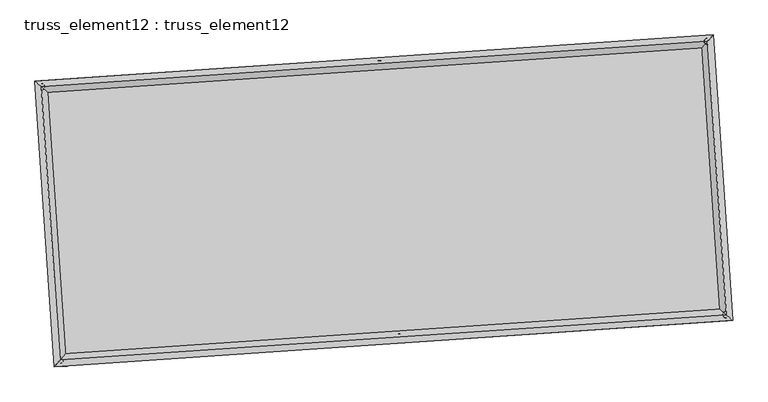
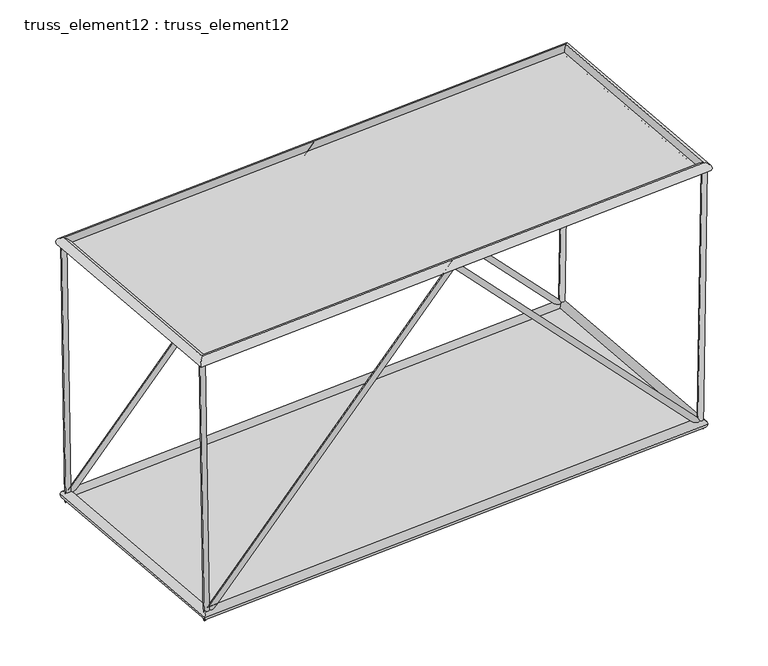
"""IFC4 building model written with IfcOpenShell, lengths in millimetres: plate geometry, truss_element12 : truss_element12."""

from ifc_helpers import new_model, si_unit, frame, origin, origin_with_axes, place, context, project, spatial, polyline, circle_curve, ellipse_curve, outline, extrude, source, transform, mapped, element, save
from ifc_brep_helpers import plane_surface, cylinder_surface, advanced_brep


def truss_element12_truss_element12_e04a6144(model_context):
    return source(origin(), model_context, "Body", "SolidModel", [
        advanced_brep(
        [(-3747.6745809, 2270.5827391, 5000.1397912), (-3846.7642532, 2257.2224013, 4998.4850332), (-3666.955388, 2276.0866741, 122.1016657), (-3762.0314948, 2263.000006, -122.1016657), (1063.0159613, 2598.6054401, 5071.4427914), (1063.4746685, 2592.0329278, 4927.2050516), (5794.3605037, 2921.2178389, 122.1113555), (5890.4004734, 2921.1626496, -122.1113555), (5873.7167781, 2926.6288416, 5000.1488436), (5973.7033156, 2926.8427538, 4998.522018)],
        [
            (0, 1, circle_curve(frame((-3797.2194171, 2263.9025702, 4999.3124122), z_axis=(-0.016545195126705874, -0.0011281539615153604, 0.9998624824378892), x_axis=(-0.13360367338721058, 0.9910342399034762, -0.0010926098951407265)), 50.0)),
            (1, 0, circle_curve(frame((-3797.2194171, 2263.9025702, 4999.3124122), z_axis=(-0.016545195126705874, -0.0011281539615153604, 0.9998624824378892), x_axis=(-0.13360367338721058, 0.9910342399034762, -0.0010926098951407265)), 50.0)),
            (0, 2),
            (2, 3, ellipse_curve(frame((-3714.4934414, 2269.54334, 0.0), z_axis=(-0.9288422213363263, -0.06333422021308809, 0.36502178621693154), x_axis=(0.36417617531422575, 0.024831789031433106, 0.9309989772212431)), 131.4368172, 50.0)),
            (3, 1),
            (3, 2, ellipse_curve(frame((-3714.4934414, 2269.54334, 0.0), z_axis=(-0.9288422213363263, -0.06333422021308809, 0.36502178621693154), x_axis=(0.36417617531422575, 0.024831789031433106, 0.9309989772212431)), 131.4368172, 50.0)),
            (2, 4),
            (4, 5, ellipse_curve(frame((1063.2453149, 2595.319184, 4999.3239215), z_axis=(-0.997683393417191, -0.06802823804748823, -7.299118212962024e-05), x_axis=(7.282209047061573e-05, 4.965461526506492e-06, -0.9999999973361438)), 72.2759091, 50.0)),
            (5, 3),
            (5, 4, ellipse_curve(frame((1063.2453149, 2595.319184, 4999.3239215), z_axis=(-0.997683393417191, -0.06802823804748823, -7.299118212962024e-05), x_axis=(7.282209047061573e-05, 4.965461526506492e-06, -0.9999999973361438)), 72.2759091, 50.0)),
            (4, 6),
            (6, 7, ellipse_curve(frame((5842.3804885, 2921.1902443, 0.0), z_axis=(-0.9287646394568846, -0.06332893019964528, -0.3652200584500962), x_axis=(-0.36437398822915673, -0.024845277142144923, 0.9309212151979933)), 131.4582279, 50.0)),
            (7, 5),
            (7, 6, ellipse_curve(frame((5842.3804885, 2921.1902443, 0.0), z_axis=(-0.9287646394568846, -0.06332893019964528, -0.3652200584500962), x_axis=(-0.36437398822915673, -0.024845277142144923, 0.9309212151979933)), 131.4582279, 50.0)),
            (8, 9, circle_curve(frame((5923.7100469, 2926.7357977, 4999.3354308), z_axis=(0.01626591167596563, 0.0011091106846651945, 0.9998670861623753), x_axis=(-0.0021568808380560416, 0.9999970970113657, -0.001074166603327577)), 50.0)),
            (9, 8, circle_curve(frame((5923.7100469, 2926.7357977, 4999.3354308), z_axis=(0.01626591167596563, 0.0011091106846651945, 0.9998670861623753), x_axis=(-0.0021568808380560416, 0.9999970970113657, -0.001074166603327577)), 50.0)),
            (6, 8),
            (9, 7),
        ],
        [
            plane_surface(frame((-3797.2194171, 2313.9025384, 4999.3688276), z_axis=(-0.016545195126705083, -0.0011281539615101183, 0.9998624824378892), x_axis=(0.9998631188908906, -1.8668082733874755e-05, 0.0165451845950244))),
            cylinder_surface(frame((-3797.2194171, 2263.9025702, 4999.3124122), z_axis=(-0.016545195126705874, -0.0011281539615153604, 0.9998624824378892), x_axis=(-0.13360367338721058, 0.9910342399034762, -0.0010926098951407265)), 50.0),
            cylinder_surface(frame((-3714.4934414, 2269.54334, 0.0), z_axis=(-0.6901382450820989, -0.04705790347107508, -0.7221459384334359), x_axis=(-0.020412126279864194, 0.9987523412193734, -0.045575278491254055)), 50.0),
            cylinder_surface(frame((1063.2453149, 2595.319184, 4999.3239215), z_axis=(-0.6902434140818253, -0.04706507454538159, 0.7220449487910731), x_axis=(-0.1153420922788449, 0.9922794277004869, -0.04558222363084794)), 50.0),
            plane_surface(frame((5923.7100469, 2876.7358284, 4999.3908937), z_axis=(0.016265911675964573, 0.001109110684661795, 0.9998670861623755), x_axis=(0.9998677013072028, -1.8043083512608863e-05, -0.016265901668749198))),
            cylinder_surface(frame((5842.3804885, 2921.1902443, 0.0), z_axis=(-0.01626591167596563, -0.0011091106846651945, -0.9998670861623753), x_axis=(-0.0021568808380560416, 0.9999970970113657, -0.001074166603327577)), 50.0),
        ],
        [
            (0, [[1, 2]]),
            (1, [[-1, 3, 4, 5]]),
            (1, [[-2, -5, 6, -3]]),
            (2, [[-4, 7, 8, 9]]),
            (2, [[-6, -9, 10, -7]]),
            (3, [[-8, 11, 12, 13]]),
            (3, [[-10, -13, 14, -11]]),
            (4, [[15, 16]]),
            (5, [[-12, 17, -16, 18]]),
            (5, [[-14, -18, -15, -17]]),
        ],
    ),
        advanced_brep(
        [(-3475.561628, -1720.1508452, 5000.1397912), (-3574.6513003, -1733.511183, 4998.4850332), (-3394.8424351, -1714.6469102, 122.1016657), (-3489.9185419, -1727.7335783, -122.1016657), (1335.1289143, -1392.1281442, 5071.4427914), (1335.5876214, -1398.7006565, 4927.2050516), (6066.4734566, -1069.5157454, 122.1113555), (6162.5134263, -1069.5709347, -122.1113555), (6145.829731, -1064.1047427, 5000.1488436), (6245.8162685, -1063.8908305, 4998.522018)],
        [
            (0, 1, circle_curve(frame((-3525.1064641, -1726.8310141, 4999.3124122), z_axis=(-0.016545195126705655, -0.0011281539615153268, 0.9998624824378892), x_axis=(-0.13360367338721035, 0.9910342399034762, -0.0010926098951407272)), 50.0)),
            (1, 0, circle_curve(frame((-3525.1064641, -1726.8310141, 4999.3124122), z_axis=(-0.016545195126705655, -0.0011281539615153268, 0.9998624824378892), x_axis=(-0.13360367338721035, 0.9910342399034762, -0.0010926098951407272)), 50.0)),
            (0, 2),
            (2, 3, ellipse_curve(frame((-3442.3804885, -1721.1902443, 0.0), z_axis=(-0.9288422213363263, -0.06333422021308796, 0.3650217862169315), x_axis=(0.3641761753142257, 0.024831789031433064, 0.930998977221243)), 131.4368172, 50.0)),
            (3, 1),
            (3, 2, ellipse_curve(frame((-3442.3804885, -1721.1902443, 0.0), z_axis=(-0.9288422213363263, -0.06333422021308796, 0.3650217862169315), x_axis=(0.3641761753142257, 0.024831789031433064, 0.930998977221243)), 131.4368172, 50.0)),
            (2, 4),
            (4, 5, ellipse_curve(frame((1335.3582678, -1395.4144003, 4999.3239215), z_axis=(-0.997683393417191, -0.06802823804748816, -7.299118212962024e-05), x_axis=(7.282209047061571e-05, 4.9654615265353194e-06, -0.9999999973361438)), 72.2759091, 50.0)),
            (5, 3),
            (5, 4, ellipse_curve(frame((1335.3582678, -1395.4144003, 4999.3239215), z_axis=(-0.997683393417191, -0.06802823804748816, -7.299118212962024e-05), x_axis=(7.282209047061571e-05, 4.9654615265353194e-06, -0.9999999973361438)), 72.2759091, 50.0)),
            (4, 6),
            (6, 7, ellipse_curve(frame((6114.4934414, -1069.54334, 0.0), z_axis=(-0.9287646394568848, -0.06332893019964522, -0.3652200584500961), x_axis=(-0.3643739882291565, -0.024845277142144934, 0.9309212151979933)), 131.4582279, 50.0)),
            (7, 5),
            (7, 6, ellipse_curve(frame((6114.4934414, -1069.54334, 0.0), z_axis=(-0.9287646394568848, -0.06332893019964522, -0.3652200584500961), x_axis=(-0.3643739882291565, -0.024845277142144934, 0.9309212151979933)), 131.4582279, 50.0)),
            (8, 9, circle_curve(frame((6195.8229998, -1063.9977866, 4999.3354308), z_axis=(0.01626591167596574, 0.0011091106846651574, 0.9998670861623753), x_axis=(-0.002156880838055875, 0.9999970970113657, -0.0010741666033275423)), 50.0)),
            (9, 8, circle_curve(frame((6195.8229998, -1063.9977866, 4999.3354308), z_axis=(0.01626591167596574, 0.0011091106846651574, 0.9998670861623753), x_axis=(-0.002156880838055875, 0.9999970970113657, -0.0010741666033275423)), 50.0)),
            (6, 8),
            (9, 7),
        ],
        [
            plane_surface(frame((-3525.1064641, -1676.8310459, 4999.3688276), z_axis=(-0.016545195126705083, -0.0011281539615101122, 0.9998624824378892), x_axis=(0.9998631188908906, -1.8668082733874755e-05, 0.0165451845950244))),
            cylinder_surface(frame((-3525.1064641, -1726.8310141, 4999.3124122), z_axis=(-0.016545195126705655, -0.0011281539615153268, 0.9998624824378892), x_axis=(-0.13360367338721035, 0.9910342399034762, -0.0010926098951407272)), 50.0),
            cylinder_surface(frame((-3442.3804885, -1721.1902443, 0.0), z_axis=(-0.690138245082099, -0.04705790347107502, -0.722145938433436), x_axis=(-0.020412126279864152, 0.9987523412193734, -0.045575278491254)), 50.0),
            cylinder_surface(frame((1335.3582678, -1395.4144003, 4999.3239215), z_axis=(-0.6902434140818253, -0.0470650745453816, 0.7220449487910733), x_axis=(-0.11534209227884486, 0.9922794277004869, -0.04558222363084788)), 50.0),
            plane_surface(frame((6195.8229998, -1113.9977559, 4999.3908937), z_axis=(0.016265911675964573, 0.0011091106846617862, 0.9998670861623755), x_axis=(0.9998677013072028, -1.8043083512164774e-05, -0.016265901668749198))),
            cylinder_surface(frame((6114.4934414, -1069.54334, 0.0), z_axis=(-0.01626591167596574, -0.0011091106846651574, -0.9998670861623753), x_axis=(-0.002156880838055875, 0.9999970970113657, -0.0010741666033275423)), 50.0),
        ],
        [
            (0, [[1, 2]]),
            (1, [[-1, 3, 4, 5]]),
            (1, [[-2, -5, 6, -3]]),
            (2, [[-4, 7, 8, 9]]),
            (2, [[-6, -9, 10, -7]]),
            (3, [[-8, 11, 12, 13]]),
            (3, [[-10, -13, 14, -11]]),
            (4, [[15, 16]]),
            (5, [[-12, 17, -16, 18]]),
            (5, [[-14, -18, -15, -17]]),
        ],
    ),
        advanced_brep(
        [(-3525.1004475, -1726.8243456, 4909.3124124), (-3525.1124808, -1726.8376825, 5089.312412), (-3797.2262832, 2263.9083603, 5089.312412), (-3797.2125509, 2263.8967802, 4909.3124124), (5923.7156393, 2926.7424372, 5089.3354306), (5923.7044545, 2926.7291581, 4909.335431), (6195.8294417, -1064.0036056, 5089.3354306), (6195.8165579, -1063.9919676, 4909.335431)],
        [
            (0, 1, ellipse_curve(frame((-3525.1064641, -1726.8310141, 4999.3124122), z_axis=(-0.7535719234034888, 0.6573654662782155, -1.6705107863312232e-06), x_axis=(-0.6573654662761124, -0.7535719234053234, -1.6705107863314445e-06)), 127.2792206, 90.0)),
            (1, 2),
            (2, 3, ellipse_curve(frame((-3797.2194171, 2263.9025702, 4999.3124122), z_axis=(-0.6573654662761124, -0.7535719234053236, -1.6705107863316489e-06), x_axis=(0.7535719234034892, -0.657365466278215, 1.670510786331429e-06)), 127.2792206, 90.0)),
            (3, 0),
            (1, 0, ellipse_curve(frame((-3525.1064641, -1726.8310141, 4999.3124122), z_axis=(-0.7535719234034888, 0.6573654662782155, -1.6705107863312232e-06), x_axis=(-0.6573654662761124, -0.7535719234053234, -1.6705107863314445e-06)), 127.2792206, 90.0)),
            (3, 2, ellipse_curve(frame((-3797.2194171, 2263.9025702, 4999.3124122), z_axis=(-0.6573654662761124, -0.7535719234053236, -1.6705107863316489e-06), x_axis=(0.7535719234034892, -0.657365466278215, 1.670510786331429e-06)), 127.2792206, 90.0)),
            (2, 4),
            (4, 5, ellipse_curve(frame((5923.7100469, 2926.7357977, 4999.3354308), z_axis=(-0.7535719234034889, 0.6573654662782153, -1.6705107863316334e-06), x_axis=(-0.6573654662761127, -0.7535719234053232, -1.6705107863314443e-06)), 127.2792206, 90.0)),
            (5, 3),
            (5, 4, ellipse_curve(frame((5923.7100469, 2926.7357977, 4999.3354308), z_axis=(-0.7535719234034889, 0.6573654662782153, -1.6705107863316334e-06), x_axis=(-0.6573654662761127, -0.7535719234053232, -1.6705107863314443e-06)), 127.2792206, 90.0)),
            (4, 6),
            (6, 7, ellipse_curve(frame((6195.8229998, -1063.9977866, 4999.3354308), z_axis=(0.6573654662761125, 0.7535719234053233, 1.670510786331239e-06), x_axis=(-0.7535719234034888, 0.6573654662782155, -1.6705107863314284e-06)), 127.2792206, 90.0)),
            (7, 5),
            (7, 6, ellipse_curve(frame((6195.8229998, -1063.9977866, 4999.3354308), z_axis=(0.6573654662761125, 0.7535719234053233, 1.670510786331239e-06), x_axis=(-0.7535719234034888, 0.6573654662782155, -1.6705107863314284e-06)), 127.2792206, 90.0)),
            (6, 1),
            (0, 7),
        ],
        [
            cylinder_surface(frame((-3525.1064641, -1726.8310141, 4999.3124122), z_axis=(0.06802823822870091, -0.9976833960748768, 0.0), x_axis=(-0.9976833935077207, -0.0680282380536563, -7.173725476018443e-05)), 90.0),
            cylinder_surface(frame((-3797.2194171, 2263.9025702, 4999.3124122), z_axis=(-0.9976833960720924, -0.06802823822851116, -2.3624590101206056e-06), x_axis=(-0.0680282379014803, 0.9976833936851697, -6.937479575574905e-05)), 90.0),
            cylinder_surface(frame((5923.7100469, 2926.7357977, 4999.3354308), z_axis=(-0.06802823822870059, 0.9976833960748767, 0.0), x_axis=(0.9976833938347516, 0.06802823807595497, -6.70123367513137e-05)), 90.0),
            cylinder_surface(frame((6195.8229998, -1063.9977866, 4999.3354308), z_axis=(0.9976833960720927, 0.06802823822851081, 2.3624590101203164e-06), x_axis=(0.06802823822851081, -0.9976833936628708, -6.937479575574907e-05)), 90.0),
        ],
        [
            (0, [[1, 2, 3, 4]]),
            (0, [[5, -4, 6, -2]]),
            (1, [[-3, 7, 8, 9]]),
            (1, [[-6, -9, 10, -7]]),
            (2, [[-8, 11, 12, 13]]),
            (2, [[-10, -13, 14, -11]]),
            (3, [[-12, 15, -1, 16]]),
            (3, [[-14, -16, -5, -15]]),
        ],
    ),
        advanced_brep(
        [(-3358.7115243, -1625.2761972, 0.0), (-3526.0494527, -1817.1042913, 0.0), (-3810.4074885, 2353.2123043, 0.0), (-3618.5793943, 2185.8743758, 0.0), (5926.0494527, 3017.1042913, 0.0), (5758.7115243, 2825.2761972, 0.0), (6210.4074885, -1153.2123043, 0.0), (6018.5793943, -985.8743758, 0.0)],
        [
            (0, 1, ellipse_curve(frame((-3442.3804885, -1721.1902443, 0.0), z_axis=(-0.7535719234054609, 0.6573654662780776, 0.0), x_axis=(-0.6573654662780776, -0.7535719234054606, 0.0)), 127.2792206, 90.0)),
            (1, 2),
            (2, 3, ellipse_curve(frame((-3714.4934414, 2269.54334, 0.0), z_axis=(-0.6573654662780776, -0.7535719234054609, 0.0), x_axis=(0.7535719234054609, -0.6573654662780776, 0.0)), 127.2792206, 90.0)),
            (3, 0),
            (1, 0, ellipse_curve(frame((-3442.3804885, -1721.1902443, 0.0), z_axis=(-0.7535719234054609, 0.6573654662780776, 0.0), x_axis=(-0.6573654662780776, -0.7535719234054606, 0.0)), 127.2792206, 90.0)),
            (3, 2, ellipse_curve(frame((-3714.4934414, 2269.54334, 0.0), z_axis=(-0.6573654662780776, -0.7535719234054609, 0.0), x_axis=(0.7535719234054609, -0.6573654662780776, 0.0)), 127.2792206, 90.0)),
            (2, 4),
            (4, 5, ellipse_curve(frame((5842.3804885, 2921.1902443, 0.0), z_axis=(-0.7535719234054609, 0.6573654662780776, 0.0), x_axis=(-0.6573654662780775, -0.7535719234054609, 0.0)), 127.2792206, 90.0)),
            (5, 3),
            (5, 4, ellipse_curve(frame((5842.3804885, 2921.1902443, 0.0), z_axis=(-0.7535719234054609, 0.6573654662780776, 0.0), x_axis=(-0.6573654662780775, -0.7535719234054609, 0.0)), 127.2792206, 90.0)),
            (4, 6),
            (6, 7, ellipse_curve(frame((6114.4934414, -1069.54334, 0.0), z_axis=(0.6573654662780776, 0.7535719234054609, 0.0), x_axis=(-0.753571923405461, 0.6573654662780775, 0.0)), 127.2792206, 90.0)),
            (7, 5),
            (7, 6, ellipse_curve(frame((6114.4934414, -1069.54334, 0.0), z_axis=(0.6573654662780776, 0.7535719234054609, 0.0), x_axis=(-0.753571923405461, 0.6573654662780775, 0.0)), 127.2792206, 90.0)),
            (6, 1),
            (0, 7),
        ],
        [
            cylinder_surface(frame((-3442.3804885, -1721.1902443, 0.0), z_axis=(0.0680282382287054, -0.9976833960748763, 0.0), x_axis=(-0.9976833960748763, -0.0680282382287054, 0.0)), 90.0),
            cylinder_surface(frame((-3714.4934414, 2269.54334, 0.0), z_axis=(-0.9976833960748763, -0.0680282382287058, 0.0), x_axis=(-0.0680282382287058, 0.9976833960748763, 0.0)), 90.0),
            cylinder_surface(frame((5842.3804885, 2921.1902443, 0.0), z_axis=(-0.06802823822870546, 0.9976833960748763, 0.0), x_axis=(0.9976833960748763, 0.06802823822870546, 0.0)), 90.0),
            cylinder_surface(frame((6114.4934414, -1069.54334, 0.0), z_axis=(0.9976833960748763, 0.06802823822870585, 0.0), x_axis=(0.06802823822870585, -0.9976833960748763, 0.0)), 90.0),
        ],
        [
            (0, [[1, 2, 3, 4]]),
            (0, [[5, -4, 6, -2]]),
            (1, [[-3, 7, 8, 9]]),
            (1, [[-6, -9, 10, -7]]),
            (2, [[-8, 11, 12, 13]]),
            (2, [[-10, -13, 14, -11]]),
            (3, [[-12, 15, -1, 16]]),
            (3, [[-14, -16, -5, -15]]),
        ],
    ),
        extrude(outline(polyline([(-3442.3804885, -1721.1902443), (-3714.4934414, 2269.54334), (5842.3804885, 2921.1902443), (6114.4934414, -1069.54334), (-3442.3804885, -1721.1902443)])), origin_with_axes(), (0.0, 0.0, 1.0), 20.0),
        extrude(outline(polyline([(-2000.0, 4871.7506486), (2000.0, 4871.7506487), (2000.0, -4871.7506486), (-2000.0, -4871.7506486), (-2000.0, 4871.7506486)])), frame((1199.3017914, 599.9523918, 4999.3239215), z_axis=(-2.3569861283046724e-06, -1.6071392434602567e-07, 0.9999999999972095), x_axis=(-0.06802823822870514, 0.9976833960748763, 0.0)), (0.0, 0.0, 1.0), 20.0),
    ])


if __name__ == "__main__":
    model = new_model("IFC4")
    model_context = context("Model", 3, world=origin())
    ifc_project = project(units=[si_unit("LENGTHUNIT", "METRE", prefix="MILLI")], contexts=[model_context])
    site = spatial("IfcSite", under=ifc_project)
    building = spatial("IfcBuilding", under=site)
    placement = place(None, origin())
    truss_element12_truss_element12_shape = truss_element12_truss_element12_e04a6144(model_context)
    element("IfcPlate", 1, ObjectType="truss_element12 : truss_element12", at=placement, inside=building, context=model_context, shape_type="MappedRepresentation", body=[
        mapped(truss_element12_truss_element12_shape, transform((0.0, 0.0, 0.0), x_axis=(1.0, 0.0, 0.0), y_axis=(0.0, 1.0, 0.0), z_axis=(0.0, 0.0, 1.0))),
    ])
    save(model, "model.ifc")

# Revit data of these elements
# Type "truss_element12 : truss_element12"
#   steellbar1 = 90 mm
#   steelbar2 = 50 mm
#   offset1 = 5000 mm
#   M = Default Roof
# Element 1 (IfcPlate, "truss_element12 : truss_element12")
#   Materials on its faces: "Default Roof"
# Materials
#   "Default Roof": class "Miscellaneous", colour RGB 0 127 0, transparency 0, Comments = "Rendering appearance not upgraded Rendering appearance not upgraded ", Cost = 0
